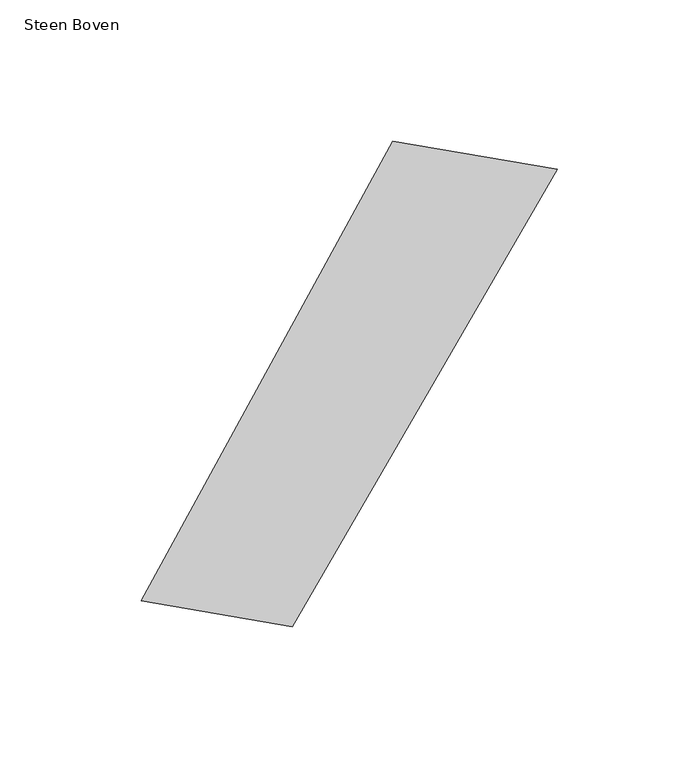
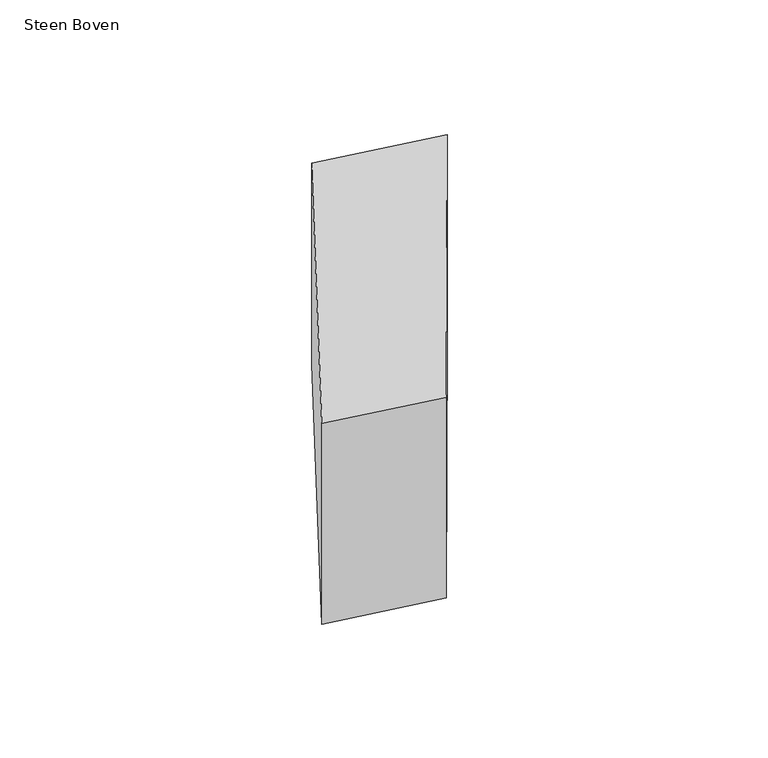
"""IFC4 building model written with IfcOpenShell, lengths in millimetres: proxy geometry, 00_GMA_steen_versie_4 : Steen Boven."""

from ifc_helpers import new_model, si_unit, origin, origin_with_axes, place, context, project, spatial, polyline, outline, extrude, source, transform, mapped, element, save


def steen_boven_7310186c(model_context):
    return source(origin(), model_context, "Body", "SweptSolid", [
        extrude(outline(polyline([(148.8055175, 152.5156886), (54.9522509, -9.3122663), (1.614426, -0.1736166), (90.6804944, 162.4360672), (148.8055175, 152.5156886)])), origin_with_axes(), (0.0, 0.0, 1.0), 100.0),
    ])


if __name__ == "__main__":
    model = new_model("IFC4")
    model_context = context("Model", 3, world=origin())
    ifc_project = project(units=[si_unit("LENGTHUNIT", "METRE", prefix="MILLI")], contexts=[model_context])
    site = spatial("IfcSite", under=ifc_project)
    building = spatial("IfcBuilding", under=site)
    placement = place(None, origin())
    steen_boven_shape = steen_boven_7310186c(model_context)
    element("IfcBuildingElementProxy", 1, Name="00_GMA_steen_versie_4 : Steen Boven", ObjectType="00_GMA_steen_versie_4 : Steen Boven", at=placement, inside=building, context=model_context, shape_type="MappedRepresentation", body=[
        mapped(steen_boven_shape, transform((0.0, 0.0, 0.0), x_axis=(1.0, 0.0, 0.0), y_axis=(0.0, 1.0, 0.0), z_axis=(0.0, 0.0, 1.0))),
    ])
    save(model, "model.ifc")

# Revit data of these elements
# Type "00_GMA_steen_versie_4 : Steen Boven"
#   StootVoegHalfBoven [instance default] = 5 mm
#   StootVoegHalf [instance default] = 5 mm
#   StootVoegBreedteOnder = 10 mm
#   StootVoegBreedteBoven = 10 mm
#   Steendikte = 100 mm
#   LintVoegOnderHalf = 5 mm
#   LintVoegOnder = 10 mm
#   LintVoegBovenHalf = 0 mm
#   LintVoegBoven = 0 mm
#   materiaal = none
#   MateriaalVoeg = none
#   Default Elevation = 0
